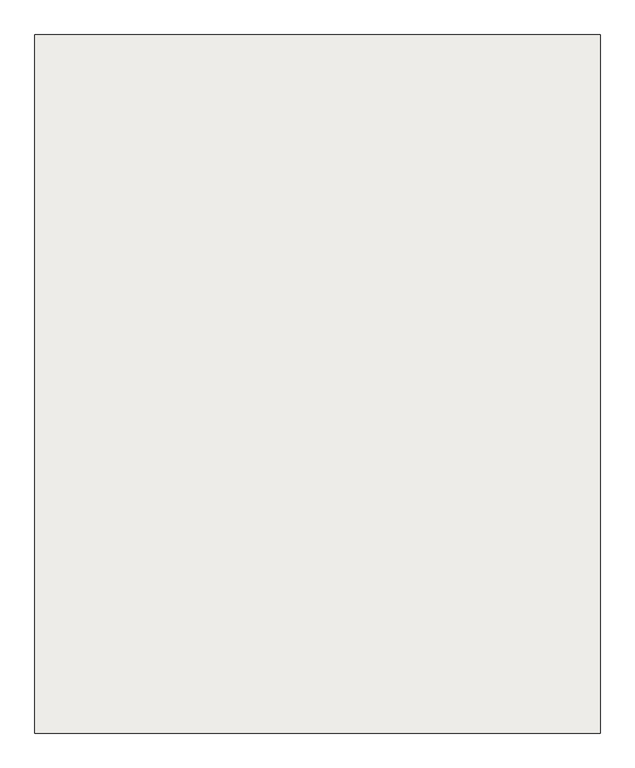
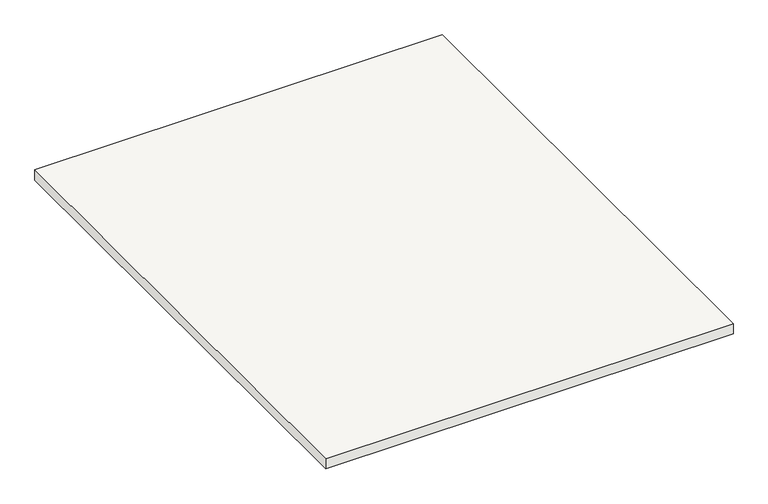
"""IFC4 building model written with IfcOpenShell, lengths in millimetres: slab geometry, Holzdecke 176 : Holzdecke 176."""

from ifc_helpers import new_model, si_unit, frame, origin, place, context, project, spatial, polyline, outline, extrude, source, transform, mapped, element, save


def slab_4f2d1623(model_context):
    return source(origin(), model_context, "Body", "SweptSolid", [
        extrude(outline(polyline([(174297.7593015, 47984.7962965), (174297.7593015, 26981.9343946), (157297.7593015, 26981.9343946), (157297.7593015, 47984.7962965), (174297.7593015, 47984.7962965)])), frame((0.0, 0.0, 2880.0), z_axis=(0.0, 0.0, 1.0), x_axis=(1.0, 0.0, 0.0)), (0.0, 0.0, 1.0), 450.0),
    ])


if __name__ == "__main__":
    model = new_model("IFC4")
    model_context = context("Model", 3, world=origin())
    ifc_project = project(units=[si_unit("LENGTHUNIT", "METRE", prefix="MILLI")], contexts=[model_context])
    site = spatial("IfcSite", under=ifc_project)
    building = spatial("IfcBuilding", under=site)
    placement = place(None, origin())
    slab_shape = slab_4f2d1623(model_context)
    element("IfcSlab", 1, ObjectType="Holzdecke 176 : Holzdecke 176", at=placement, inside=building, context=model_context, shape_type="MappedRepresentation", body=[
        mapped(slab_shape, transform((0.0, 0.0, 0.0), x_axis=(1.0, 0.0, 0.0), y_axis=(0.0, 1.0, 0.0), z_axis=(0.0, 0.0, 1.0))),
    ])
    save(model, "model.ifc")

# Revit data of these elements
# Type "Holzdecke 176 : Holzdecke 176"
#   Abrechnungsart = "m²"
#   Allright_Bauteil_ID = "0113De 0783954357"
#   Bezeichnung = "Holzdecke"
#   Codetext = "D-HOLZBALKEN1\\"
#   Gewerk = "Zimmer- und Holzbauarbeiten"
#   Material = "Holz"
#   Objektname = "Brettstapeldecke"
#   NameOverride = "Holzdecke"
#   Reference = "Holzdecke"
#   Status = "NEW"
#   PitchAngle = 0.00°
#   ThermalTransmittance = 0.0000 BTU/(h·ft²·°F)
#   2D Interaktion = yes
#   Combustible = no
#   Compartmentation = no
#   IsExternal = no
#   LoadBearing = yes
# Element 1 (IfcSlab, "Holzdecke 176 : Holzdecke 176")
#   Materials on its faces: "holzschalung"
# Materials
#   "holzschalung": class "Unassigned", colour RGB 128 128 128, transparency 0
